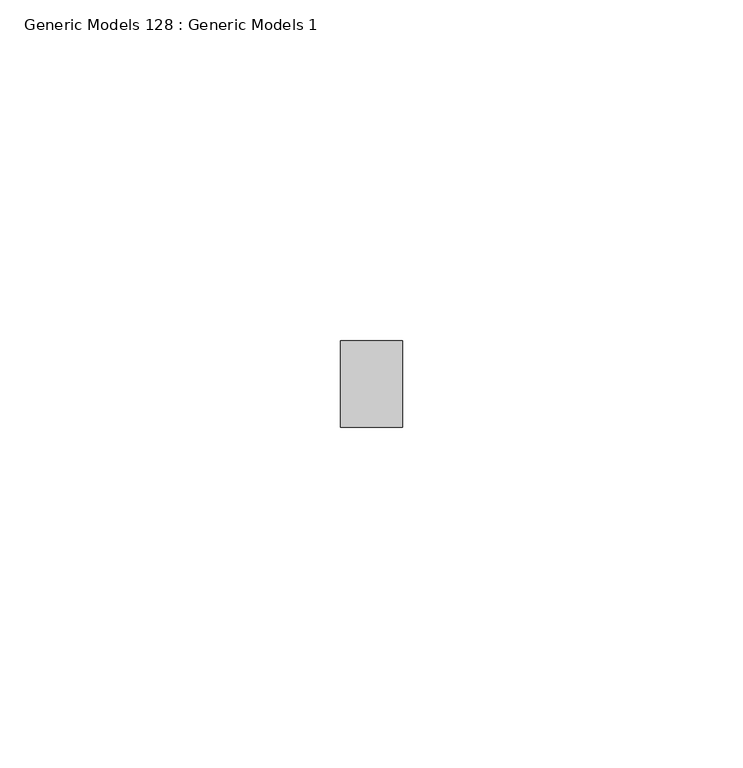
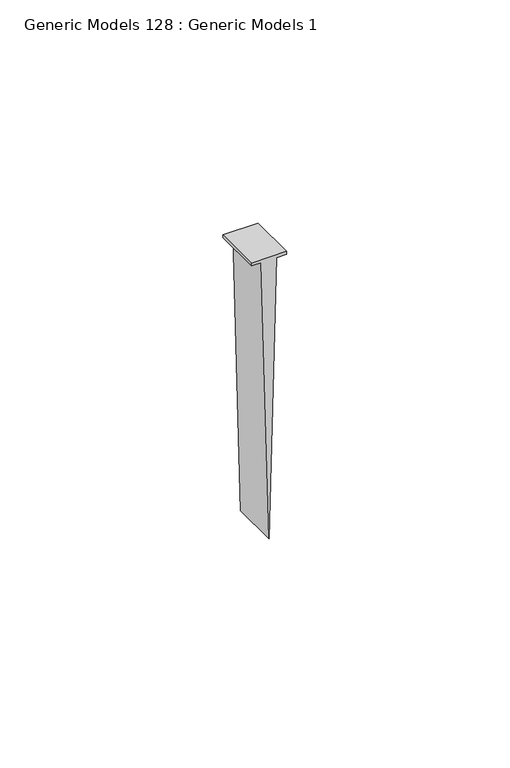
"""IFC4 building model written with IfcOpenShell, lengths in millimetres: proxy geometry, Generic Models 128 : Generic Models 1."""

from ifc_helpers import new_model, si_unit, frame, origin, place, context, project, spatial, polyline, outline, extrude, source, transform, mapped, element, save


def generic_models_128_generic_models_1_f3b2dce0(model_context):
    return source(origin(), model_context, "Body", "SweptSolid", [
        extrude(outline(polyline([(2443.027413, 49845.474547), (2442.233663, 49845.474547), (2442.233663, 49848.0244106), (2366.033663, 49850.021147), (2442.233663, 49852.0178834), (2442.233663, 49854.567747), (2443.027413, 49854.567747), (2443.027413, 49845.474547)])), frame((0.0, 565.15, 0.0), z_axis=(0.0, 1.0, 0.0), x_axis=(0.0, 0.0, 1.0)), (0.0, 0.0, 1.0), 12.7),
    ])


if __name__ == "__main__":
    model = new_model("IFC4")
    model_context = context("Model", 3, world=origin())
    ifc_project = project(units=[si_unit("LENGTHUNIT", "METRE", prefix="MILLI")], contexts=[model_context])
    site = spatial("IfcSite", under=ifc_project)
    building = spatial("IfcBuilding", under=site)
    placement = place(None, origin())
    generic_models_128_generic_models_1_shape = generic_models_128_generic_models_1_f3b2dce0(model_context)
    element("IfcBuildingElementProxy", 1, Name="Generic Models 128 : Generic Models 1", ObjectType="Generic Models 128 : Generic Models 1", at=placement, inside=building, context=model_context, shape_type="MappedRepresentation", body=[
        mapped(generic_models_128_generic_models_1_shape, transform((0.0, 0.0, 0.0), x_axis=(1.0, 0.0, 0.0), y_axis=(0.0, 1.0, 0.0), z_axis=(0.0, 0.0, 1.0))),
    ])
    save(model, "model.ifc")

# Revit data of these elements
# Element 1 (IfcBuildingElementProxy, "Generic Models 128 : Generic Models 1")
#   Materials on its faces: "ATTACH GYPSUM BOARD TO STUDS AND NOT TO TOP TRACK"
# Materials
#   "ATTACH GYPSUM BOARD TO STUDS AND NOT TO TOP TRACK": class "Generic", colour RGB 48 48 48, transparency 0, Cost = 0
